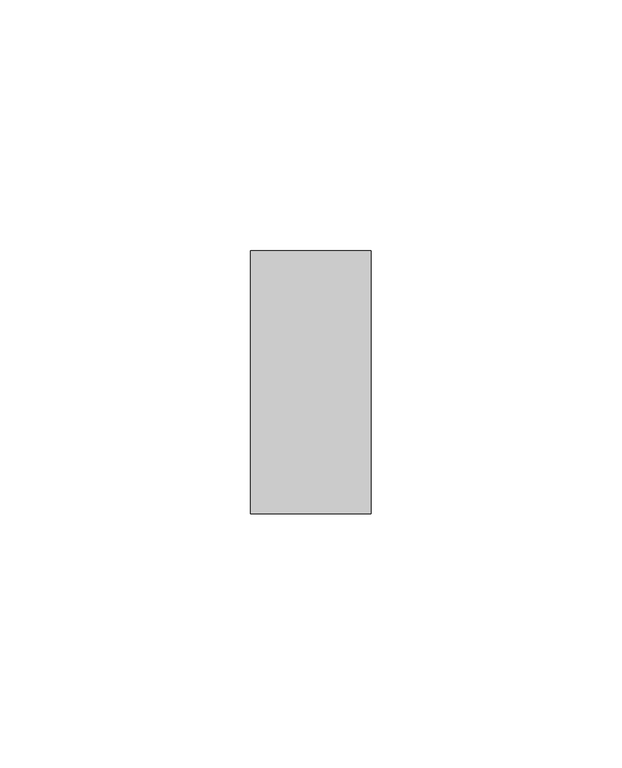
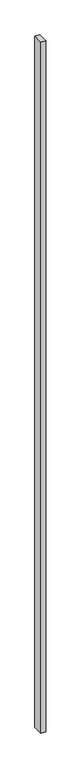
"""IFC4 building model written with IfcOpenShell, lengths in millimetres: proxy geometry, Generic Models 11:Generic Models 1:306267:Generic Models 1:306267 : Generic Models 11:Generic Models 1:306267:300405:Generic Models 1:306267:Generic Models 1:306267 : Generic Models 11:Generic Models 1:306267:300405 : Generic Models 11:Generic Models 1:306267:Generic Models 1:306267 : Generic Models 11:Generic Models 1:306267:300405:17 : Generic Models 11:Generic Models 1:306267:Generic Models 1:306267 : Generic Models 11:Generic Models 1:306267:300405:Generic Models 1:306267:Generic Models 1:306267 : Generic Models 11:Generic Models 1:306267:300405 : Generic Models 11:Generic Models 1:306267:Generic Models 1:306267 : Generic Models 11:Generic Models 1:306267:300405:300182."""

from ifc_helpers import new_model, si_unit, origin, origin_with_axes, place, context, project, spatial, polyline, outline, extrude, source, transform, mapped, element, save


def generic_models_e469c9c7(model_context):
    return source(origin(), model_context, "Body", "SweptSolid", [
        extrude(outline(polyline([(593733.0974915, -579018.6137729), (593757.1367239, -579018.6137729), (593757.1367239, -579071.0475719), (593733.0974915, -579071.0475719), (593733.0974915, -579018.6137729)])), origin_with_axes(), (0.0, 0.0, 1.0), 3702.05),
    ])


if __name__ == "__main__":
    model = new_model("IFC4")
    model_context = context("Model", 3, world=origin())
    ifc_project = project(units=[si_unit("LENGTHUNIT", "METRE", prefix="MILLI")], contexts=[model_context])
    site = spatial("IfcSite", under=ifc_project)
    building = spatial("IfcBuilding", under=site)
    placement = place(None, origin())
    generic_models_shape = generic_models_e469c9c7(model_context)
    element("IfcBuildingElementProxy", 1, Name="Generic Models 11:Generic Models 1:306267:Generic Models 1:306267 : Generic Models 11:Generic Models 1:306267:300405:Generic Models 1:306267:Generic Models 1:306267 : Generic Models 11:Generic Models 1:306267:300405 : Generic Models 11:Generic Models 1:306267:Generic Models 1:306267 : Generic Models 11:Generic Models 1:306267:300405:17 : Generic Models 11:Generic Models 1:306267:Generic Models 1:306267 : Generic Models 11:Generic Models 1:306267:300405:Generic Models 1:306267:Generic Models 1:306267 : Generic Models 11:Generic Models 1:306267:300405 : Generic Models 11:Generic Models 1:306267:Generic Models 1:306267 : Generic Models 11:Generic Models 1:306267:300405:300182", ObjectType="Generic Models 11:Generic Models 1:306267:Generic Models 1:306267 : Generic Models 11:Generic Models 1:306267:300405:Generic Models 1:306267:Generic Models 1:306267 : Generic Models 11:Generic Models 1:306267:300405 : Generic Models 11:Generic Models 1:306267:Generic Models 1:306267 : Generic Models 11:Generic Models 1:306267:300405:17 : Generic Models 11:Generic Models 1:306267:Generic Models 1:306267 : Generic Models 11:Generic Models 1:306267:300405:Generic Models 1:306267:Generic Models 1:306267 : Generic Models 11:Generic Models 1:306267:300405 : Generic Models 11:Generic Models 1:306267:Generic Models 1:306267 : Generic Models 11:Generic Models 1:306267:300405:300182", at=placement, inside=building, context=model_context, shape_type="MappedRepresentation", body=[
        mapped(generic_models_shape, transform((0.0, 0.0, 0.0), x_axis=(1.0, 0.0, 0.0), y_axis=(0.0, 1.0, 0.0), z_axis=(0.0, 0.0, 1.0))),
    ])
    save(model, "model.ifc")

# Revit data of these elements
# Type "Generic Models 11:Generic Models 1:306267:Generic Models 1:306267 : Generic Models 11:Generic Models 1:306267:300405:Generic Models 1:306267:Generic Models 1:306267 : Generic Models 11:Generic Models 1:306267:300405 : Generic Models 11:Generic Models 1:306267:Generic Models 1:306267 : Generic Models 11:Generic Models 1:306267:300405:17 : Generic Models 11:Generic Models 1:306267:Generic Models 1:306267 : Generic Models 11:Generic Models 1:306267:300405:Generic Models 1:306267:Generic Models 1:306267 : Generic Models 11:Generic Models 1:306267:300405 : Generic Models 11:Generic Models 1:306267:Generic Models 1:306267 : Generic Models 11:Generic Models 1:306267:300405:300182"
#   NameOverride = "Generic Models 11:Generic Models 1:306267:Generic Models 1:306267 : Generic Models 11:Generic Models 1:306267:300405:Generic Models 1:306267:Generic Models 1:306267 : Generic Models 11:Generic Models 1:306267:300405 : Generic Models 11:Generic Models 1:306267:Generic Models 1:306267 : Generic Models 11:Generic Models 1:306267:300405:300182"
#   ObjectTypeOverride = "Generic Models 1:306267:Generic Models 1:306267 : Generic Models 11:Generic Models 1:306267:300405 : Generic Models 11:Generic Models 1:306267:Generic Models 1:306267 : Generic Models 11:Generic Models 1:306267:300405"
#   Reference = "Generic Models 1"
#   Tag = "300182"
# Element 1 (IfcBuildingElementProxy, "Generic Models 11:Generic Models 1:306267:Generic Models 1:306267 : Generic Models 11:Generic Models 1:306267:300405:Generic Models 1:306267:Generic Models 1:306267 : Generic Models 11:Generic Models 1:306267:300405 : Generic Models 11:Generic Models 1:306267:Generic Models 1:306267 : Generic Models 11:Generic Models 1:306267:300405:17 : Generic Models 11:Generic Models 1:306267:Generic Models 1:306267 : Generic Models 11:Generic Models 1:306267:300405:Generic Models 1:306267:Generic Models 1:306267 : Generic Models 11:Generic Models 1:306267:300405 : Generic Models 11:Generic Models 1:306267:Generic Models 1:306267 : Generic Models 11:Generic Models 1:306267:300405:300182")
#   Materials on its faces: "PRESSURE TREATED WOOD BLOCKING - SIZE AS NECESSARY"
# Materials
#   "PRESSURE TREATED WOOD BLOCKING - SIZE AS NECESSARY": class "Wood", colour RGB 144 113 62, transparency 0, Description = "Pinus Echinata", Cost = 0
